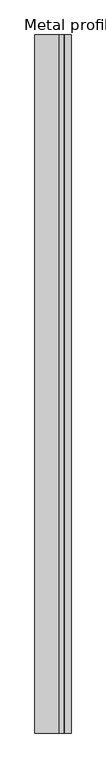
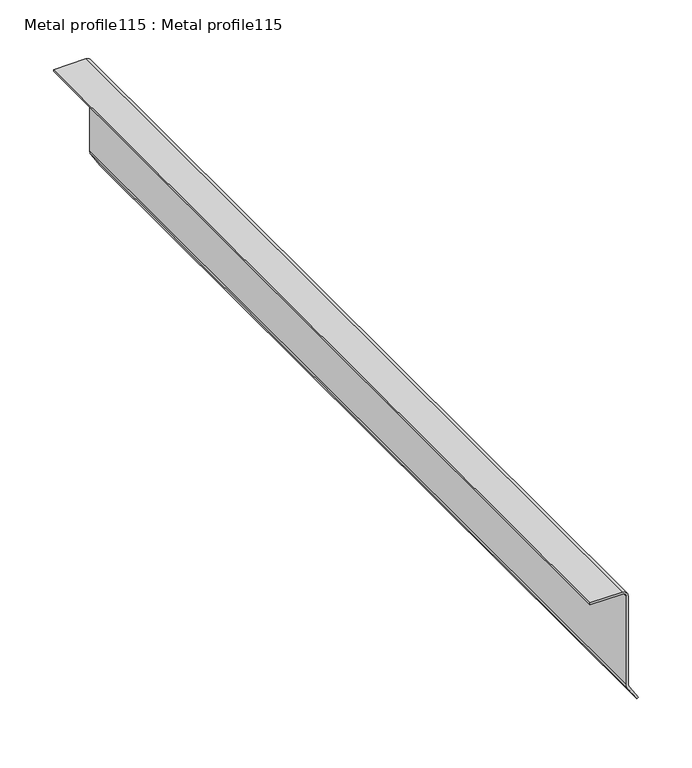
"""IFC4 building model written with IfcOpenShell, lengths in millimetres: proxy geometry, Metal profile115 : Metal profile115."""

from ifc_helpers import new_model, si_unit, point, frame, frame_2d, origin, place, context, project, spatial, polyline, circle_curve, trimmed, segment, composite_curve, outline, extrude, source, transform, mapped, element, save


def metal_profile115_metal_profile115_646f8386(model_context):
    return source(origin(), model_context, "Body", "SweptSolid", [
        extrude(outline(composite_curve([segment(polyline([(18.5969529, 1e-07), (18.5969529, -2.005263), (0.0, -2.005263)]), True, "CONTINUOUS"), segment(trimmed(circle_curve(frame_2d((-1e-07, -8.4330125)), 6.4277495), [point((0.0, -2.005263))], [point((-3.3815471, -2.9666515))], True, "CARTESIAN"), True, "CONTINUOUS"), segment(polyline([(-3.3815471, -2.9666515), (-88.3494682, -55.5286794)]), True, "CONTINUOUS"), segment(trimmed(circle_curve(frame_2d((-91.7811821, -49.9812222)), 6.5231081), [point((-88.3494682, -55.5286794))], [point((-97.3286391, -53.4129361))], False, "CARTESIAN"), True, "CONTINUOUS"), segment(polyline([(-97.3286391, -53.4129361), (-115.4703641, -24.0863534), (-113.7650251, -23.0314132), (-95.6233002, -52.3579959)]), True, "CONTINUOUS"), segment(trimmed(circle_curve(frame_2d((-91.7811821, -49.9812222)), 4.5178451), [point((-95.6233002, -52.3579959))], [point((-89.4044084, -53.8233404))], True, "CARTESIAN"), True, "CONTINUOUS"), segment(polyline([(-89.4044084, -53.8233404), (-4.4364873, -1.2613125)]), True, "CONTINUOUS"), segment(trimmed(circle_curve(frame_2d((-1e-07, -8.4330125)), 8.4330125), [point((-4.4364873, -1.2613125))], [point((0.0, 0.0))], False, "CARTESIAN"), True, "CONTINUOUS"), segment(polyline([(0.0, 0.0), (18.5969529, 1e-07)]), True, "CONTINUOUS")], self_intersect=False)), frame((-7111.9308248, 7982.1531721, 40057.7644016), z_axis=(3.673949545698047e-12, 1.0, 0.0), x_axis=(0.5260856920621059, -1.932812289349816e-12, -0.8504315637413368)), (0.0, 0.0, 1.0), 1000.0),
    ])


if __name__ == "__main__":
    model = new_model("IFC4")
    model_context = context("Model", 3, world=origin())
    ifc_project = project(units=[si_unit("LENGTHUNIT", "METRE", prefix="MILLI")], contexts=[model_context])
    site = spatial("IfcSite", under=ifc_project)
    building = spatial("IfcBuilding", under=site)
    placement = place(None, origin())
    metal_profile115_metal_profile115_shape = metal_profile115_metal_profile115_646f8386(model_context)
    element("IfcBuildingElementProxy", 1, Name="Metal profile115 : Metal profile115", ObjectType="Metal profile115 : Metal profile115", at=placement, inside=building, context=model_context, shape_type="MappedRepresentation", body=[
        mapped(metal_profile115_metal_profile115_shape, transform((0.0, 0.0, 0.0), x_axis=(1.0, 0.0, 0.0), y_axis=(0.0, 1.0, 0.0), z_axis=(0.0, 0.0, 1.0))),
    ])
    save(model, "model.ifc")

# Revit data of these elements
# Type "Metal profile115 : Metal profile115"
#   NameOverride = "Metal profile115"
# Element 1 (IfcBuildingElementProxy, "Metal profile115 : Metal profile115")
#   Materials on its faces: "ANGLE TRIM"
# Materials
#   "ANGLE TRIM": class "Unassigned", colour RGB 245 226 176, transparency 0, Cost = 0
